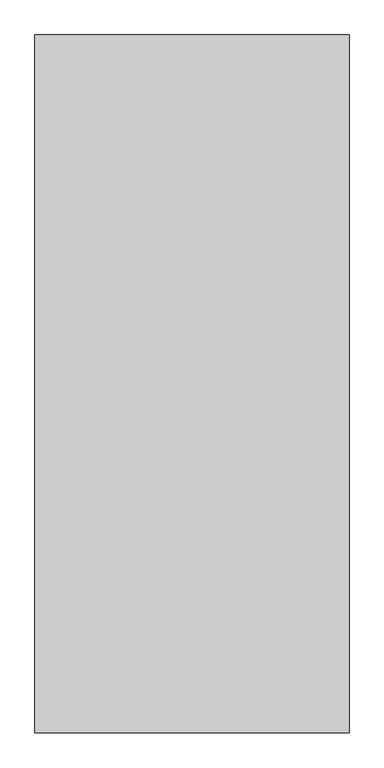
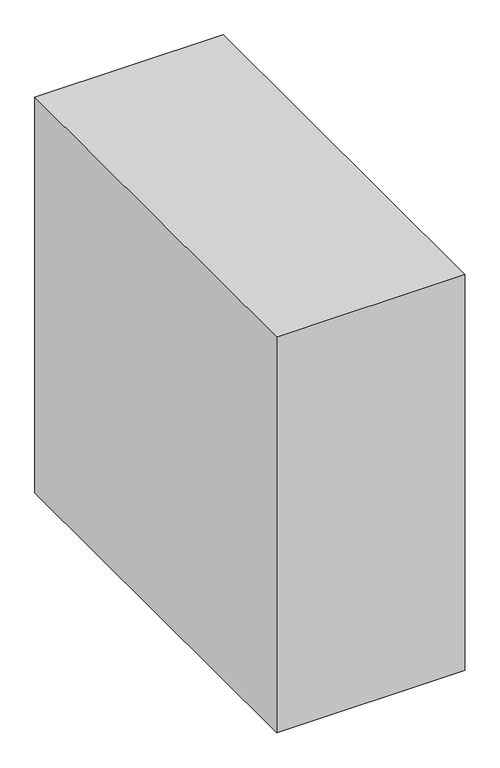
"""IFC4 building model written with IfcOpenShell, lengths in millimetres: proxy geometry, Space Planning Box_hec : Space Planning Box_hec."""

from ifc_helpers import new_model, si_unit, origin, origin_with_axes, place, context, project, spatial, polyline, outline, extrude, source, transform, mapped, element, save


def generic_models_5634f436(model_context):
    return source(origin(), model_context, "Body", "SweptSolid", [
        extrude(outline(polyline([(1350.0, 3000.0), (1350.0, -3000.0), (-1350.0, -3000.0), (-1350.0, 3000.0), (1350.0, 3000.0)])), origin_with_axes(), (0.0, 0.0, 1.0), 6000.0),
    ])


if __name__ == "__main__":
    model = new_model("IFC4")
    model_context = context("Model", 3, world=origin())
    ifc_project = project(units=[si_unit("LENGTHUNIT", "METRE", prefix="MILLI")], contexts=[model_context])
    site = spatial("IfcSite", under=ifc_project)
    building = spatial("IfcBuilding", under=site)
    placement = place(None, origin())
    generic_models_shape = generic_models_5634f436(model_context)
    element("IfcBuildingElementProxy", 1, Name="Space Planning Box_hec : Space Planning Box_hec", ObjectType="Space Planning Box_hec : Space Planning Box_hec", at=placement, inside=building, context=model_context, shape_type="MappedRepresentation", body=[
        mapped(generic_models_shape, transform((0.0, 0.0, 0.0), x_axis=(1.0, 0.0, 0.0), y_axis=(0.0, 1.0, 0.0), z_axis=(0.0, 0.0, 1.0))),
    ])
    save(model, "model.ifc")

# Revit data of these elements
# Type "Space Planning Box_hec : Space Planning Box_hec"
#   Type Comments = "..."
#   Room Name [instance default] = "?"
#   Interior Finish [instance default] = ""
#   Exterior Finish [instance default] = ""
#   Department [instance default] = ""
#   Assembly Code = "..."
#   Width [instance default] = 1524 mm
#   Program Area [instance default] = 0 m²
#   Length [instance default] = 1524 mm
#   Height [instance default] = 1524 mm
#   Area [instance default] = 2.32258 m²
#   Fill Color [instance default] = Cyan
#   Default Elevation = 0
# Element 1 (IfcBuildingElementProxy, "Space Planning Box_hec : Space Planning Box_hec")
#   Room Name = "Duct Shaft"
#   Interior Finish = "NA"
#   Exterior Finish = "EF1"
#   Department = "HV"
#   Width = 2700 mm
#   Program Area = 16.2 m²
#   Length = 6000 mm
#   Height = 6000 mm
#   Area = 16.2 m²
#   Fill Color = Pink
#   Materials on its faces: "Pink"
# Materials
#   "Cyan": class "Generic", colour RGB 0 255 255, transparency 0.2, Cost = 0
#   "Pink": class "Generic", colour RGB 255 105 180, transparency 0.2, Cost = 0
